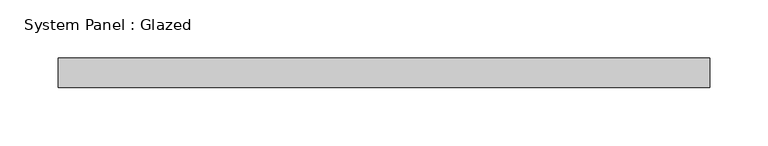
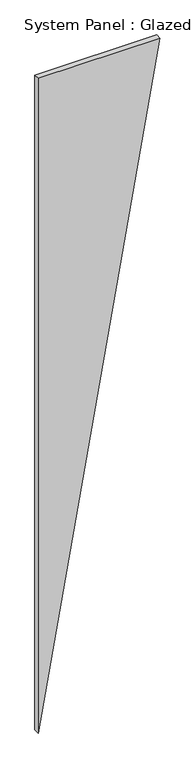
"""IFC4 building model written with IfcOpenShell, lengths in millimetres: plate geometry, System Panel : Glazed."""

import ifcopenshell
import ifcopenshell.guid

model = None  # the IFC model being written
_history = None  # IfcOwnerHistory: only IFC2X3 demands one
_inside = {}  # id of a spatial element -> (the spatial element, [elements in it])
_under = {}  # id of a project, library or spatial element -> (it, [spatial elements below it])
_declared = {}  # id of a project -> (the project, [libraries it declares])
_typed = {}  # id of a type object -> (the type object, [elements of that type])
_made_of = {}  # id of a material, layer set ... -> (it, [elements and type objects made of it])


def new_model(schema):
    """Start an empty IFC model of exactly this schema.

    Asked for "IFC4X3", IfcOpenShell would pick the latest addendum, in which some entities
    have other attributes; the version numbers below select the first issue.
    IFC2X3 requires an IfcOwnerHistory on every rooted entity: one is made here for all.
    """
    global model, _history
    if schema == "IFC4X3":
        model = ifcopenshell.file(schema_version=(4, 3, 0, 0))
    else:
        model = ifcopenshell.file(schema=schema)
    _inside.clear()
    _under.clear()
    _declared.clear()
    _typed.clear()
    _made_of.clear()
    _history = None
    if model.schema == "IFC2X3":
        org = make("IfcOrganization", Name="unknown")
        user = make(
            "IfcPersonAndOrganization",
            ThePerson=make("IfcPerson", FamilyName="unknown"),
            TheOrganization=org,
        )
        app = make(
            "IfcApplication",
            ApplicationDeveloper=org,
            Version="unknown",
            ApplicationFullName="unknown",
            ApplicationIdentifier="unknown",
        )
        _history = make(
            "IfcOwnerHistory",
            OwningUser=user,
            OwningApplication=app,
            ChangeAction="ADDED",
            CreationDate=0,
        )
    return model


def make(cls, **values):
    """One entity of the class cls with the attributes given. An attribute that is None is left unset."""
    return model.create_entity(
        cls, **{name: value for name, value in values.items() if value is not None}
    )


def rooted(cls, **values):
    """An entity with a GlobalId (a new one), such as an element, a storey or a relation."""
    return make(cls, GlobalId=ifcopenshell.guid.new(), OwnerHistory=_history, **values)


def si_unit(unit_type, name, prefix=None):
    """IfcSIUnit, for example si_unit("LENGTHUNIT", "METRE", prefix="MILLI")."""
    return make("IfcSIUnit", UnitType=unit_type, Prefix=prefix, Name=name)


def assignment(units):
    """IfcUnitAssignment: the units of a project."""
    return None if units is None else make("IfcUnitAssignment", Units=units)


def point(xyz):
    """IfcCartesianPoint."""
    return None if xyz is None else make("IfcCartesianPoint", Coordinates=xyz)


def direction(xyz):
    """IfcDirection."""
    return None if xyz is None else make("IfcDirection", DirectionRatios=xyz)


def frame(location, z_axis=None, x_axis=None):
    """IfcAxis2Placement3D, a coordinate frame: its origin and axes. An axis left out is left unset."""
    return make(
        "IfcAxis2Placement3D",
        Location=point(location),
        Axis=direction(z_axis),
        RefDirection=direction(x_axis),
    )


def origin():
    """The frame at (0, 0, 0) with its axes left unset."""
    return frame((0.0, 0.0, 0.0))


def place(relative_to, where):
    """IfcLocalPlacement: puts the frame where relative to a parent placement (None: the world)."""
    return make(
        "IfcLocalPlacement", PlacementRelTo=relative_to, RelativePlacement=where
    )


def context(
    kind, dimensions, precision=None, world=None, true_north=None, identifier=None
):
    """IfcGeometricRepresentationContext, for example the 3D "Model" context."""
    return make(
        "IfcGeometricRepresentationContext",
        ContextIdentifier=identifier,
        ContextType=kind,
        CoordinateSpaceDimension=dimensions,
        Precision=precision,
        WorldCoordinateSystem=world,
        TrueNorth=true_north,
    )


def project(units=None, contexts=None):
    """IfcProject with its units and contexts."""
    return rooted(
        "IfcProject",
        Name="project",
        RepresentationContexts=contexts,
        UnitsInContext=assignment(units),
    )


def spatial(cls, under=None, at=None, **own):
    """A site, building, storey or space (cls), placed at a placement, below another one or the project."""
    s = rooted(cls, ObjectPlacement=at, **own)
    if under is not None:
        _under.setdefault(under.id(), (under, []))[1].append(s)
    return s


def polyline(points):
    """IfcPolyline through the points."""
    return make("IfcPolyline", Points=[point(p) for p in points])


def outline(outer, holes=None, kind="AREA"):
    """IfcArbitraryClosedProfileDef: a profile drawn as a closed curve; with holes, ...WithVoids."""
    if holes is None:
        return make("IfcArbitraryClosedProfileDef", ProfileType=kind, OuterCurve=outer)
    return make(
        "IfcArbitraryProfileDefWithVoids",
        ProfileType=kind,
        OuterCurve=outer,
        InnerCurves=holes,
    )


def extrude(swept, where, along, depth):
    """IfcExtrudedAreaSolid: the profile swept, set in the frame where, extruded along a direction by depth."""
    return make(
        "IfcExtrudedAreaSolid",
        SweptArea=swept,
        Position=where,
        ExtrudedDirection=direction(along),
        Depth=depth,
    )


def shape(context_of_items, identifier, shape_type, items):
    """IfcShapeRepresentation: the items that make up one representation, for example the "Body"."""
    return make(
        "IfcShapeRepresentation",
        ContextOfItems=context_of_items,
        RepresentationIdentifier=identifier,
        RepresentationType=shape_type,
        Items=items,
    )


def source(mapping_origin, context_of_items, identifier, shape_type, items):
    """IfcRepresentationMap: a shape defined once, which mapped items show again and again."""
    return make(
        "IfcRepresentationMap",
        MappingOrigin=mapping_origin,
        MappedRepresentation=shape(context_of_items, identifier, shape_type, items),
    )


def transform(
    local_origin,
    x_axis=None,
    y_axis=None,
    z_axis=None,
    scale=None,
    scale2=None,
    scale3=None,
    uniform=True,
):
    """IfcCartesianTransformationOperator3D, or its non-uniform kind. x_axis, y_axis, z_axis: its Axis1, 2, 3."""
    if uniform:
        return make(
            "IfcCartesianTransformationOperator3D",
            Axis1=direction(x_axis),
            Axis2=direction(y_axis),
            LocalOrigin=point(local_origin),
            Scale=scale,
            Axis3=direction(z_axis),
        )
    return make(
        "IfcCartesianTransformationOperator3DnonUniform",
        Axis1=direction(x_axis),
        Axis2=direction(y_axis),
        LocalOrigin=point(local_origin),
        Scale=scale,
        Axis3=direction(z_axis),
        Scale2=scale2,
        Scale3=scale3,
    )


def mapped(mapping_source, mapping_target):
    """IfcMappedItem: shows the shape of a source again, moved by a transform."""
    return make(
        "IfcMappedItem", MappingSource=mapping_source, MappingTarget=mapping_target
    )


def made_of(thing, what):
    """Note that an element or type object is made of a material, layer set ...; save() writes the relation."""
    if what is not None:
        _made_of.setdefault(what.id(), (what, []))[1].append(thing)
    return thing


def element(
    cls,
    number,
    at=None,
    inside=None,
    cuts=None,
    type_object=None,
    material=None,
    context=None,
    identifier="Body",
    shape_type=None,
    held_by="IfcProductDefinitionShape",
    body=None,
    shapes=None,
    **own,
):
    """One element of the class cls, such as IfcWall. Its Tag is "e" and its number.

    at: its placement. inside: the storey or other place that contains it. cuts: it is an
    opening in that element (IfcRelVoidsElement). A single representation is given by context,
    identifier, shape_type and body (its items); several are given by shapes. held_by: the class
    of the entity that holds the representations. save() writes the other relations.
    """
    e = rooted(cls, Tag="e%d" % number, ObjectPlacement=at, **own)
    if body is not None:
        shapes = [shape(context, identifier, shape_type, body)]
    if shapes is not None:
        e.Representation = make(held_by, Representations=shapes)
    if inside is not None:
        _inside.setdefault(inside.id(), (inside, []))[1].append(e)
    if cuts is not None:
        rooted(
            "IfcRelVoidsElement", RelatingBuildingElement=cuts, RelatedOpeningElement=e
        )
    if type_object is not None:
        _typed.setdefault(type_object.id(), (type_object, []))[1].append(e)
    return made_of(e, material)


def aggregate(whole, parts):
    """IfcRelAggregates: a whole, such as a stair, and the parts it consists of."""
    return rooted("IfcRelAggregates", RelatingObject=whole, RelatedObjects=parts)


def save(model, path):
    """Write the relations noted so far, then the file.

    IfcRelAggregates (storeys below a building ...), IfcRelContainedInSpatialStructure (elements
    in a storey), IfcRelDefinesByType, IfcRelAssociatesMaterial and IfcRelDeclares: one each for
    every whole, place, type object, material and project.
    """
    for whole, parts in _under.values():
        aggregate(whole, parts)
    for where, things in _inside.values():
        rooted(
            "IfcRelContainedInSpatialStructure",
            RelatedElements=things,
            RelatingStructure=where,
        )
    for kind, things in _typed.values():
        rooted("IfcRelDefinesByType", RelatedObjects=things, RelatingType=kind)
    for what, things in _made_of.values():
        rooted("IfcRelAssociatesMaterial", RelatedObjects=things, RelatingMaterial=what)
    for by, libraries in _declared.values():
        rooted("IfcRelDeclares", RelatingContext=by, RelatedDefinitions=libraries)
    model.write(path)


def system_panel_glazed_04b02cc8(model_context):
    return source(origin(), model_context, "Body", "SweptSolid", [
        extrude(outline(polyline([(0.0, -280.4314386), (3192.9616215, 280.4314386), (3192.9616215, -280.4314386), (0.0, -280.4314386)])), frame((0.0, -44.45, 0.0), z_axis=(0.0, 1.0, 0.0), x_axis=(0.0, 0.0, 1.0)), (0.0, 0.0, 1.0), 25.4),
    ])


if __name__ == "__main__":
    model = new_model("IFC4")
    model_context = context("Model", 3, world=origin())
    ifc_project = project(units=[si_unit("LENGTHUNIT", "METRE", prefix="MILLI")], contexts=[model_context])
    site = spatial("IfcSite", under=ifc_project)
    building = spatial("IfcBuilding", under=site)
    placement = place(None, origin())
    system_panel_glazed_shape = system_panel_glazed_04b02cc8(model_context)
    element("IfcPlate", 1, ObjectType="System Panel : Glazed", at=placement, inside=building, context=model_context, shape_type="MappedRepresentation", body=[
        mapped(system_panel_glazed_shape, transform((0.0, 0.0, 0.0), x_axis=(1.0, 0.0, 0.0), y_axis=(0.0, 1.0, 0.0), z_axis=(0.0, 0.0, 1.0))),
    ])
    save(model, "model.ifc")

# Revit data of these elements
# Type "System Panel : Glazed"
#   Construction Type Id = "GSP4R"
#   Analytic Construction = "1/8 in Pilkington single glazing"
#   Visual Light Transmittance = 0.9
#   Solar Heat Gain Coefficient = 0.86
#   Heat Transfer Coefficient (U) = 1.18115 BTU/(h·ft²·°F)
#   Define Thermal Properties by = 1
# Element 1 (IfcPlate, "System Panel : Glazed")
#   Materials on its faces: "Glass"
# Materials
#   "Glass": class "Glass", colour RGB 0 128 192, transparency 0.75, Description = "Soda Lime Glass", Cost = 0
